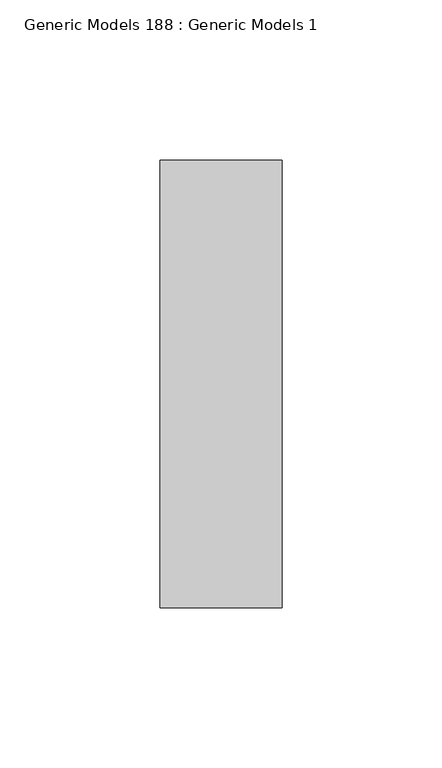
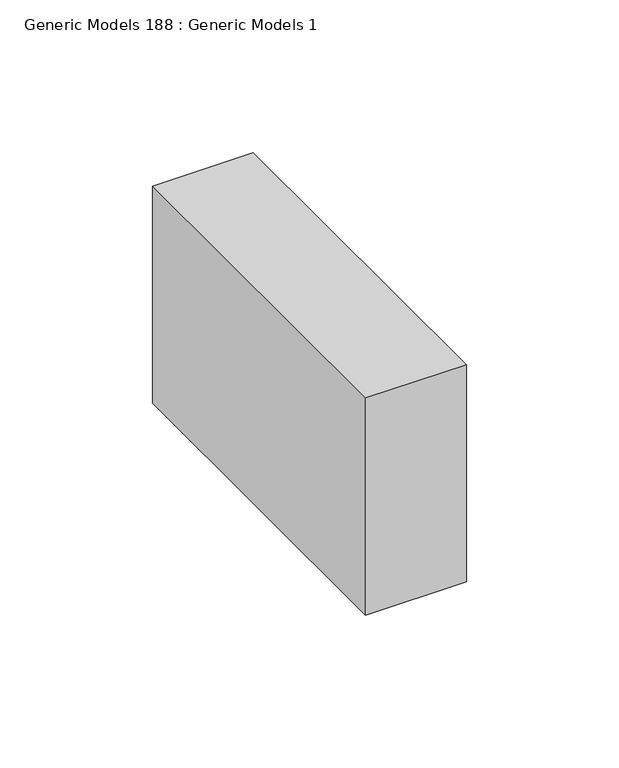
"""IFC4 building model written with IfcOpenShell, lengths in millimetres: proxy geometry, Generic Models 188 : Generic Models 1."""

from ifc_helpers import new_model, si_unit, frame, origin, place, context, project, spatial, polyline, outline, extrude, source, transform, mapped, element, save


def generic_models_188_generic_models_1_9e8f1c67(model_context):
    return source(origin(), model_context, "Body", "SweptSolid", [
        extrude(outline(polyline([(-2894.120657, -5645.2125551), (-2932.220657, -5645.2125551), (-2932.220657, -5505.5125551), (-2894.120657, -5505.5125551), (-2894.120657, -5645.2125551)])), frame((0.0, 0.0, 126809.5635), z_axis=(0.0, 0.0, 1.0), x_axis=(1.0, 0.0, 0.0)), (0.0, 0.0, 1.0), 86.963165),
    ])


if __name__ == "__main__":
    model = new_model("IFC4")
    model_context = context("Model", 3, world=origin())
    ifc_project = project(units=[si_unit("LENGTHUNIT", "METRE", prefix="MILLI")], contexts=[model_context])
    site = spatial("IfcSite", under=ifc_project)
    building = spatial("IfcBuilding", under=site)
    placement = place(None, origin())
    generic_models_188_generic_models_1_shape = generic_models_188_generic_models_1_9e8f1c67(model_context)
    element("IfcBuildingElementProxy", 1, Name="Generic Models 188 : Generic Models 1", ObjectType="Generic Models 188 : Generic Models 1", at=placement, inside=building, context=model_context, shape_type="MappedRepresentation", body=[
        mapped(generic_models_188_generic_models_1_shape, transform((0.0, 0.0, 0.0), x_axis=(1.0, 0.0, 0.0), y_axis=(0.0, 1.0, 0.0), z_axis=(0.0, 0.0, 1.0))),
    ])
    save(model, "model.ifc")

# Revit data of these elements
# Element 1 (IfcBuildingElementProxy, "Generic Models 188 : Generic Models 1")
#   Materials on its faces: "_2X BLOCKING AS REQUIRED"
# Materials
#   "_2X BLOCKING AS REQUIRED": class "Generic", colour RGB 177 130 114, transparency 0, Cost = 0
